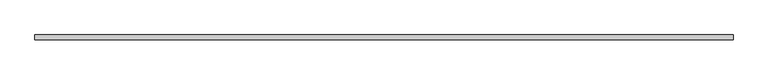
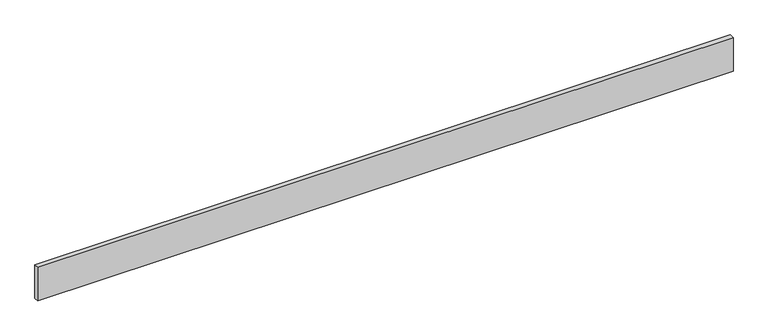
"""IFC4 building model written with IfcOpenShell, lengths in millimetres: proxy geometry, Footer001 482 : Footer001 482."""

from ifc_helpers import new_model, si_unit, frame, origin, place, context, project, spatial, polyline, outline, extrude, source, transform, mapped, element, save


def generic_models_e7b959a7(model_context):
    return source(origin(), model_context, "Body", "SweptSolid", [
        extrude(outline(polyline([(3694.2883192, 9562.5711354), (3694.2883192, 9576.3500834), (5694.2883192, 9576.3500834), (5694.2883192, 9562.5711354), (3694.2883192, 9562.5711354)])), frame((0.0, 0.0, 36582.096), z_axis=(0.0, 0.0, 1.0), x_axis=(1.0, 0.0, 0.0)), (0.0, 0.0, 1.0), 101.6),
    ])


if __name__ == "__main__":
    model = new_model("IFC4")
    model_context = context("Model", 3, world=origin())
    ifc_project = project(units=[si_unit("LENGTHUNIT", "METRE", prefix="MILLI")], contexts=[model_context])
    site = spatial("IfcSite", under=ifc_project)
    building = spatial("IfcBuilding", under=site)
    placement = place(None, origin())
    generic_models_shape = generic_models_e7b959a7(model_context)
    element("IfcBuildingElementProxy", 1, Name="Footer001 482 : Footer001 482", ObjectType="Footer001 482 : Footer001 482", at=placement, inside=building, context=model_context, shape_type="MappedRepresentation", body=[
        mapped(generic_models_shape, transform((0.0, 0.0, 0.0), x_axis=(1.0, 0.0, 0.0), y_axis=(0.0, 1.0, 0.0), z_axis=(0.0, 0.0, 1.0))),
    ])
    save(model, "model.ifc")

# Revit data of these elements
# Type "Footer001 482 : Footer001 482"
#   NameOverride = "Footer001"
# Element 1 (IfcBuildingElementProxy, "Footer001 482 : Footer001 482")
#   Materials on its faces: "FOOTER MATERIAL TBD"
# Materials
#   "FOOTER MATERIAL TBD": class "Unassigned", colour RGB 148 103 60, transparency 0
